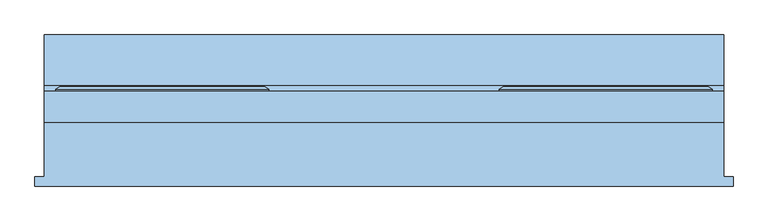
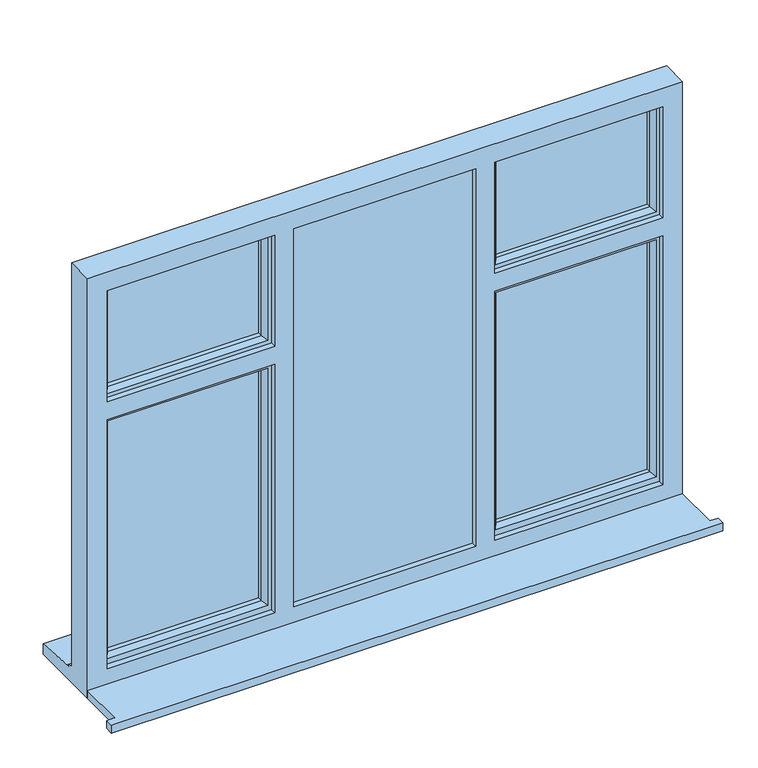
"""IFC4 building model written with IfcOpenShell, lengths in millimetres: window geometry, Window - Triple Casement with Top and Side Sashes : Window - Triple Casement with Top and Side Sashes."""

import ifcopenshell
import ifcopenshell.guid

model = None  # the IFC model being written
_history = None  # IfcOwnerHistory: only IFC2X3 demands one
_inside = {}  # id of a spatial element -> (the spatial element, [elements in it])
_under = {}  # id of a project, library or spatial element -> (it, [spatial elements below it])
_declared = {}  # id of a project -> (the project, [libraries it declares])
_typed = {}  # id of a type object -> (the type object, [elements of that type])
_made_of = {}  # id of a material, layer set ... -> (it, [elements and type objects made of it])


def new_model(schema):
    """Start an empty IFC model of exactly this schema.

    Asked for "IFC4X3", IfcOpenShell would pick the latest addendum, in which some entities
    have other attributes; the version numbers below select the first issue.
    IFC2X3 requires an IfcOwnerHistory on every rooted entity: one is made here for all.
    """
    global model, _history
    if schema == "IFC4X3":
        model = ifcopenshell.file(schema_version=(4, 3, 0, 0))
    else:
        model = ifcopenshell.file(schema=schema)
    _inside.clear()
    _under.clear()
    _declared.clear()
    _typed.clear()
    _made_of.clear()
    _history = None
    if model.schema == "IFC2X3":
        org = make("IfcOrganization", Name="unknown")
        user = make(
            "IfcPersonAndOrganization",
            ThePerson=make("IfcPerson", FamilyName="unknown"),
            TheOrganization=org,
        )
        app = make(
            "IfcApplication",
            ApplicationDeveloper=org,
            Version="unknown",
            ApplicationFullName="unknown",
            ApplicationIdentifier="unknown",
        )
        _history = make(
            "IfcOwnerHistory",
            OwningUser=user,
            OwningApplication=app,
            ChangeAction="ADDED",
            CreationDate=0,
        )
    return model


def make(cls, **values):
    """One entity of the class cls with the attributes given. An attribute that is None is left unset."""
    return model.create_entity(
        cls, **{name: value for name, value in values.items() if value is not None}
    )


def rooted(cls, **values):
    """An entity with a GlobalId (a new one), such as an element, a storey or a relation."""
    return make(cls, GlobalId=ifcopenshell.guid.new(), OwnerHistory=_history, **values)


def si_unit(unit_type, name, prefix=None):
    """IfcSIUnit, for example si_unit("LENGTHUNIT", "METRE", prefix="MILLI")."""
    return make("IfcSIUnit", UnitType=unit_type, Prefix=prefix, Name=name)


def assignment(units):
    """IfcUnitAssignment: the units of a project."""
    return None if units is None else make("IfcUnitAssignment", Units=units)


def point(xyz):
    """IfcCartesianPoint."""
    return None if xyz is None else make("IfcCartesianPoint", Coordinates=xyz)


def direction(xyz):
    """IfcDirection."""
    return None if xyz is None else make("IfcDirection", DirectionRatios=xyz)


def frame(location, z_axis=None, x_axis=None):
    """IfcAxis2Placement3D, a coordinate frame: its origin and axes. An axis left out is left unset."""
    return make(
        "IfcAxis2Placement3D",
        Location=point(location),
        Axis=direction(z_axis),
        RefDirection=direction(x_axis),
    )


def origin():
    """The frame at (0, 0, 0) with its axes left unset."""
    return frame((0.0, 0.0, 0.0))


def place(relative_to, where):
    """IfcLocalPlacement: puts the frame where relative to a parent placement (None: the world)."""
    return make(
        "IfcLocalPlacement", PlacementRelTo=relative_to, RelativePlacement=where
    )


def context(
    kind, dimensions, precision=None, world=None, true_north=None, identifier=None
):
    """IfcGeometricRepresentationContext, for example the 3D "Model" context."""
    return make(
        "IfcGeometricRepresentationContext",
        ContextIdentifier=identifier,
        ContextType=kind,
        CoordinateSpaceDimension=dimensions,
        Precision=precision,
        WorldCoordinateSystem=world,
        TrueNorth=true_north,
    )


def project(units=None, contexts=None):
    """IfcProject with its units and contexts."""
    return rooted(
        "IfcProject",
        Name="project",
        RepresentationContexts=contexts,
        UnitsInContext=assignment(units),
    )


def spatial(cls, under=None, at=None, **own):
    """A site, building, storey or space (cls), placed at a placement, below another one or the project."""
    s = rooted(cls, ObjectPlacement=at, **own)
    if under is not None:
        _under.setdefault(under.id(), (under, []))[1].append(s)
    return s


def polyline(points):
    """IfcPolyline through the points."""
    return make("IfcPolyline", Points=[point(p) for p in points])


def outline(outer, holes=None, kind="AREA"):
    """IfcArbitraryClosedProfileDef: a profile drawn as a closed curve; with holes, ...WithVoids."""
    if holes is None:
        return make("IfcArbitraryClosedProfileDef", ProfileType=kind, OuterCurve=outer)
    return make(
        "IfcArbitraryProfileDefWithVoids",
        ProfileType=kind,
        OuterCurve=outer,
        InnerCurves=holes,
    )


def extrude(swept, where, along, depth):
    """IfcExtrudedAreaSolid: the profile swept, set in the frame where, extruded along a direction by depth."""
    return make(
        "IfcExtrudedAreaSolid",
        SweptArea=swept,
        Position=where,
        ExtrudedDirection=direction(along),
        Depth=depth,
    )


def faces_of(points, faces, orient=None, outer=None):
    """IfcFace entities. A face is a list of loops; a loop is a list of indices into points, from 0.

    orient and outer hold one flag for each loop. By default every Orientation is true, the
    first loop of a face is its IfcFaceOuterBound and the others are IfcFaceBound.
    """
    made = []
    for i, loops in enumerate(faces):
        bounds = []
        for j, loop in enumerate(loops):
            is_outer = j == 0 if outer is None else outer[i][j]
            bounds.append(
                make(
                    "IfcFaceOuterBound" if is_outer else "IfcFaceBound",
                    Bound=make("IfcPolyLoop", Polygon=[points[k] for k in loop]),
                    Orientation=True if orient is None else orient[i][j],
                )
            )
        made.append(make("IfcFace", Bounds=bounds))
    return made


def faceted_brep(points, faces, orient=None, outer=None, voids=None):
    """IfcFacetedBrep: a solid bounded by flat faces; with voids (closed shells), ...WithVoids."""
    shared = [point(p) for p in points]
    hull = make("IfcClosedShell", CfsFaces=faces_of(shared, faces, orient, outer))
    if voids is None:
        return make("IfcFacetedBrep", Outer=hull)
    return make(
        "IfcFacetedBrepWithVoids",
        Outer=hull,
        Voids=[
            make(cls, CfsFaces=faces_of(shared, fs, o, b)) for cls, fs, o, b in voids
        ],
    )


def shape(context_of_items, identifier, shape_type, items):
    """IfcShapeRepresentation: the items that make up one representation, for example the "Body"."""
    return make(
        "IfcShapeRepresentation",
        ContextOfItems=context_of_items,
        RepresentationIdentifier=identifier,
        RepresentationType=shape_type,
        Items=items,
    )


def source(mapping_origin, context_of_items, identifier, shape_type, items):
    """IfcRepresentationMap: a shape defined once, which mapped items show again and again."""
    return make(
        "IfcRepresentationMap",
        MappingOrigin=mapping_origin,
        MappedRepresentation=shape(context_of_items, identifier, shape_type, items),
    )


def transform(
    local_origin,
    x_axis=None,
    y_axis=None,
    z_axis=None,
    scale=None,
    scale2=None,
    scale3=None,
    uniform=True,
):
    """IfcCartesianTransformationOperator3D, or its non-uniform kind. x_axis, y_axis, z_axis: its Axis1, 2, 3."""
    if uniform:
        return make(
            "IfcCartesianTransformationOperator3D",
            Axis1=direction(x_axis),
            Axis2=direction(y_axis),
            LocalOrigin=point(local_origin),
            Scale=scale,
            Axis3=direction(z_axis),
        )
    return make(
        "IfcCartesianTransformationOperator3DnonUniform",
        Axis1=direction(x_axis),
        Axis2=direction(y_axis),
        LocalOrigin=point(local_origin),
        Scale=scale,
        Axis3=direction(z_axis),
        Scale2=scale2,
        Scale3=scale3,
    )


def mapped(mapping_source, mapping_target):
    """IfcMappedItem: shows the shape of a source again, moved by a transform."""
    return make(
        "IfcMappedItem", MappingSource=mapping_source, MappingTarget=mapping_target
    )


def made_of(thing, what):
    """Note that an element or type object is made of a material, layer set ...; save() writes the relation."""
    if what is not None:
        _made_of.setdefault(what.id(), (what, []))[1].append(thing)
    return thing


def element(
    cls,
    number,
    at=None,
    inside=None,
    cuts=None,
    type_object=None,
    material=None,
    context=None,
    identifier="Body",
    shape_type=None,
    held_by="IfcProductDefinitionShape",
    body=None,
    shapes=None,
    **own,
):
    """One element of the class cls, such as IfcWall. Its Tag is "e" and its number.

    at: its placement. inside: the storey or other place that contains it. cuts: it is an
    opening in that element (IfcRelVoidsElement). A single representation is given by context,
    identifier, shape_type and body (its items); several are given by shapes. held_by: the class
    of the entity that holds the representations. save() writes the other relations.
    """
    e = rooted(cls, Tag="e%d" % number, ObjectPlacement=at, **own)
    if body is not None:
        shapes = [shape(context, identifier, shape_type, body)]
    if shapes is not None:
        e.Representation = make(held_by, Representations=shapes)
    if inside is not None:
        _inside.setdefault(inside.id(), (inside, []))[1].append(e)
    if cuts is not None:
        rooted(
            "IfcRelVoidsElement", RelatingBuildingElement=cuts, RelatedOpeningElement=e
        )
    if type_object is not None:
        _typed.setdefault(type_object.id(), (type_object, []))[1].append(e)
    return made_of(e, material)


def aggregate(whole, parts):
    """IfcRelAggregates: a whole, such as a stair, and the parts it consists of."""
    return rooted("IfcRelAggregates", RelatingObject=whole, RelatedObjects=parts)


def save(model, path):
    """Write the relations noted so far, then the file.

    IfcRelAggregates (storeys below a building ...), IfcRelContainedInSpatialStructure (elements
    in a storey), IfcRelDefinesByType, IfcRelAssociatesMaterial and IfcRelDeclares: one each for
    every whole, place, type object, material and project.
    """
    for whole, parts in _under.values():
        aggregate(whole, parts)
    for where, things in _inside.values():
        rooted(
            "IfcRelContainedInSpatialStructure",
            RelatedElements=things,
            RelatingStructure=where,
        )
    for kind, things in _typed.values():
        rooted("IfcRelDefinesByType", RelatedObjects=things, RelatingType=kind)
    for what, things in _made_of.values():
        rooted("IfcRelAssociatesMaterial", RelatedObjects=things, RelatingMaterial=what)
    for by, libraries in _declared.values():
        rooted("IfcRelDeclares", RelatingContext=by, RelatedDefinitions=libraries)
    model.write(path)


def window_e8f23823(model_context):
    return source(origin(), model_context, "Body", "SolidModel", [
        extrude(outline(polyline([(-1506.6666667, -182.7934322), (-1506.6666667, -157.7934322), (-1481.6666667, -157.7934322), (-1481.6666667, -13.2934322), (328.3333333, -13.2934322), (328.3333333, -157.7934322), (353.3333333, -157.7934322), (353.3333333, -182.7934322), (-1506.6666667, -182.7934322)])), frame((0.0, 0.0, 760.0), z_axis=(0.0, 0.0, 1.0), x_axis=(1.0, 0.0, 0.0)), (0.0, 0.0, 1.0), 25.0),
        extrude(outline(polyline([(823.0, -863.3333333), (823.0, -290.0), (2070.0, -290.0), (2070.0, -863.3333333), (823.0, -863.3333333)]), holes=[polyline([(2060.0, -853.3333333), (2060.0, -300.0), (833.0, -300.0), (833.0, -853.3333333), (2060.0, -853.3333333)])]), frame((0.0, 28.7065678, 0.0), z_axis=(0.0, 1.0, 0.0), x_axis=(0.0, 0.0, 1.0)), (0.0, 0.0, 1.0), 41.0),
        faceted_brep([(-1451.6666667, 69.7065678, 2080.0), (-1451.6666667, 75.4800705, 2080.0), (-1451.6666667, 75.4800705, 1665.0), (-1451.6666667, 69.7065678, 1665.0), (-1441.6666667, 4.7065678, 2070.0), (-1441.6666667, 69.7065678, 2070.0), (-1441.6666667, 69.7065678, 1675.0), (-1441.6666667, 4.7065678, 1675.0), (-1401.6666667, 19.1994677, 2030.0), (-1411.8147044, 4.7065678, 2040.1480377), (-1411.8147044, 4.7065678, 1704.8519623), (-1401.6666667, 19.1994677, 1715.0), (-1401.6666667, 33.7065678, 2030.0), (-1401.6666667, 33.7065678, 1715.0), (-1411.6666667, 57.7065678, 2040.0), (-1411.6666667, 33.7065678, 2040.0), (-1411.6666667, 33.7065678, 1705.0), (-1411.6666667, 57.7065678, 1705.0), (-1401.6666667, 75.4800705, 2030.0), (-1401.6666667, 57.7065678, 2030.0), (-1401.6666667, 57.7065678, 1715.0), (-1401.6666667, 75.4800705, 1715.0), (-1419.1124215, 81.2535732, 2047.4457548), (-1419.1124215, 81.2535732, 1697.5542452), (-1440.882057, 81.2535732, 2069.2153903), (-1440.882057, 81.2535732, 1675.7846097), (-883.3333333, 75.4800705, 1665.0), (-883.3333333, 69.7065678, 1665.0), (-893.3333333, 69.7065678, 1675.0), (-893.3333333, 4.7065678, 1675.0), (-923.1852956, 4.7065678, 1704.8519623), (-933.3333333, 19.1994677, 1715.0), (-933.3333333, 33.7065678, 1715.0), (-923.3333333, 33.7065678, 1705.0), (-923.3333333, 57.7065678, 1705.0), (-933.3333333, 57.7065678, 1715.0), (-933.3333333, 75.4800705, 1715.0), (-915.8875785, 81.2535732, 1697.5542452), (-894.117943, 81.2535732, 1675.7846097), (-883.3333333, 75.4800705, 2080.0), (-883.3333333, 69.7065678, 2080.0), (-893.3333333, 69.7065678, 2070.0), (-893.3333333, 4.7065678, 2070.0), (-923.1852956, 4.7065678, 2040.1480377), (-933.3333333, 19.1994677, 2030.0), (-933.3333333, 33.7065678, 2030.0), (-923.3333333, 33.7065678, 2040.0), (-923.3333333, 57.7065678, 2040.0), (-933.3333333, 57.7065678, 2030.0), (-933.3333333, 75.4800705, 2030.0), (-915.8875785, 81.2535732, 2047.4457548), (-894.117943, 81.2535732, 2069.2153903)], [[[0, 1, 2, 3]], [[4, 5, 6, 7]], [[8, 9, 10, 11]], [[12, 8, 11, 13]], [[14, 15, 16, 17]], [[18, 19, 20, 21]], [[22, 18, 21, 23]], [[1, 24, 25, 2]], [[3, 2, 26, 27]], [[7, 6, 28, 29]], [[11, 10, 30, 31]], [[13, 11, 31, 32]], [[17, 16, 33, 34]], [[21, 20, 35, 36]], [[23, 21, 36, 37]], [[2, 25, 38, 26]], [[27, 26, 39, 40]], [[29, 28, 41, 42]], [[31, 30, 43, 44]], [[32, 31, 44, 45]], [[34, 33, 46, 47]], [[36, 35, 48, 49]], [[37, 36, 49, 50]], [[26, 38, 51, 39]], [[40, 39, 1, 0]], [[3, 27, 40, 0], [5, 41, 28, 6]], [[42, 41, 5, 4]], [[7, 29, 42, 4], [9, 43, 30, 10]], [[44, 43, 9, 8]], [[45, 44, 8, 12]], [[15, 46, 33, 16], [13, 32, 45, 12]], [[47, 46, 15, 14]], [[17, 34, 47, 14], [19, 48, 35, 20]], [[49, 48, 19, 18]], [[50, 49, 18, 22]], [[24, 51, 38, 25], [23, 37, 50, 22]], [[39, 51, 24, 1]]]),
        faceted_brep([(-1451.6666667, 69.7065678, 1655.0), (-1451.6666667, 75.4800705, 1655.0), (-1451.6666667, 75.4800705, 813.0), (-1451.6666667, 69.7065678, 813.0), (-1441.6666667, 4.7065678, 1645.0), (-1441.6666667, 69.7065678, 1645.0), (-1441.6666667, 69.7065678, 823.0), (-1441.6666667, 4.7065678, 823.0), (-1401.6666667, 19.1994677, 1605.0), (-1411.8147044, 4.7065678, 1615.1480377), (-1411.8147044, 4.7065678, 852.8519623), (-1401.6666667, 19.1994677, 863.0), (-1401.6666667, 33.7065678, 1605.0), (-1401.6666667, 33.7065678, 863.0), (-1411.6666667, 57.7065678, 1615.0), (-1411.6666667, 33.7065678, 1615.0), (-1411.6666667, 33.7065678, 853.0), (-1411.6666667, 57.7065678, 853.0), (-1401.6666667, 75.4800705, 1605.0), (-1401.6666667, 57.7065678, 1605.0), (-1401.6666667, 57.7065678, 863.0), (-1401.6666667, 75.4800705, 863.0), (-1419.1124215, 81.2535732, 1622.4457548), (-1419.1124215, 81.2535732, 845.5542452), (-1440.882057, 81.2535732, 1644.2153903), (-1440.882057, 81.2535732, 823.7846097), (-883.3333333, 75.4800705, 813.0), (-883.3333333, 69.7065678, 813.0), (-893.3333333, 69.7065678, 823.0), (-893.3333333, 4.7065678, 823.0), (-923.1852956, 4.7065678, 852.8519623), (-933.3333333, 19.1994677, 863.0), (-933.3333333, 33.7065678, 863.0), (-923.3333333, 33.7065678, 853.0), (-923.3333333, 57.7065678, 853.0), (-933.3333333, 57.7065678, 863.0), (-933.3333333, 75.4800705, 863.0), (-915.8875785, 81.2535732, 845.5542452), (-894.117943, 81.2535732, 823.7846097), (-883.3333333, 75.4800705, 1655.0), (-883.3333333, 69.7065678, 1655.0), (-893.3333333, 69.7065678, 1645.0), (-893.3333333, 4.7065678, 1645.0), (-923.1852956, 4.7065678, 1615.1480377), (-933.3333333, 19.1994677, 1605.0), (-933.3333333, 33.7065678, 1605.0), (-923.3333333, 33.7065678, 1615.0), (-923.3333333, 57.7065678, 1615.0), (-933.3333333, 57.7065678, 1605.0), (-933.3333333, 75.4800705, 1605.0), (-915.8875785, 81.2535732, 1622.4457548), (-894.117943, 81.2535732, 1644.2153903)], [[[0, 1, 2, 3]], [[4, 5, 6, 7]], [[8, 9, 10, 11]], [[12, 8, 11, 13]], [[14, 15, 16, 17]], [[18, 19, 20, 21]], [[22, 18, 21, 23]], [[1, 24, 25, 2]], [[3, 2, 26, 27]], [[7, 6, 28, 29]], [[11, 10, 30, 31]], [[13, 11, 31, 32]], [[17, 16, 33, 34]], [[21, 20, 35, 36]], [[23, 21, 36, 37]], [[2, 25, 38, 26]], [[27, 26, 39, 40]], [[29, 28, 41, 42]], [[31, 30, 43, 44]], [[32, 31, 44, 45]], [[34, 33, 46, 47]], [[36, 35, 48, 49]], [[37, 36, 49, 50]], [[26, 38, 51, 39]], [[40, 39, 1, 0]], [[3, 27, 40, 0], [5, 41, 28, 6]], [[42, 41, 5, 4]], [[7, 29, 42, 4], [9, 43, 30, 10]], [[44, 43, 9, 8]], [[45, 44, 8, 12]], [[15, 46, 33, 16], [13, 32, 45, 12]], [[47, 46, 15, 14]], [[17, 34, 47, 14], [19, 48, 35, 20]], [[49, 48, 19, 18]], [[50, 49, 18, 22]], [[24, 51, 38, 25], [23, 37, 50, 22]], [[39, 51, 24, 1]]]),
        faceted_brep([(-270.0, 69.7065678, 2080.0), (-270.0, 75.4800705, 2080.0), (-270.0, 75.4800705, 1665.0), (-270.0, 69.7065678, 1665.0), (-260.0, 4.7065678, 2070.0), (-260.0, 69.7065678, 2070.0), (-260.0, 69.7065678, 1675.0), (-260.0, 4.7065678, 1675.0), (-220.0, 19.1994677, 2030.0), (-230.1480377, 4.7065678, 2040.1480377), (-230.1480377, 4.7065678, 1704.8519623), (-220.0, 19.1994677, 1715.0), (-220.0, 33.7065678, 2030.0), (-220.0, 33.7065678, 1715.0), (-230.0, 57.7065678, 2040.0), (-230.0, 33.7065678, 2040.0), (-230.0, 33.7065678, 1705.0), (-230.0, 57.7065678, 1705.0), (-220.0, 75.4800705, 2030.0), (-220.0, 57.7065678, 2030.0), (-220.0, 57.7065678, 1715.0), (-220.0, 75.4800705, 1715.0), (-237.4457548, 81.2535732, 2047.4457548), (-237.4457548, 81.2535732, 1697.5542452), (-259.2153903, 81.2535732, 2069.2153903), (-259.2153903, 81.2535732, 1675.7846097), (298.3333333, 75.4800705, 1665.0), (298.3333333, 69.7065678, 1665.0), (288.3333333, 69.7065678, 1675.0), (288.3333333, 4.7065678, 1675.0), (258.4813711, 4.7065678, 1704.8519623), (248.3333333, 19.1994677, 1715.0), (248.3333333, 33.7065678, 1715.0), (258.3333333, 33.7065678, 1705.0), (258.3333333, 57.7065678, 1705.0), (248.3333333, 57.7065678, 1715.0), (248.3333333, 75.4800705, 1715.0), (265.7790881, 81.2535732, 1697.5542452), (287.5487236, 81.2535732, 1675.7846097), (298.3333333, 75.4800705, 2080.0), (298.3333333, 69.7065678, 2080.0), (288.3333333, 69.7065678, 2070.0), (288.3333333, 4.7065678, 2070.0), (258.4813711, 4.7065678, 2040.1480377), (248.3333333, 19.1994677, 2030.0), (248.3333333, 33.7065678, 2030.0), (258.3333333, 33.7065678, 2040.0), (258.3333333, 57.7065678, 2040.0), (248.3333333, 57.7065678, 2030.0), (248.3333333, 75.4800705, 2030.0), (265.7790881, 81.2535732, 2047.4457548), (287.5487236, 81.2535732, 2069.2153903)], [[[0, 1, 2, 3]], [[4, 5, 6, 7]], [[8, 9, 10, 11]], [[12, 8, 11, 13]], [[14, 15, 16, 17]], [[18, 19, 20, 21]], [[22, 18, 21, 23]], [[1, 24, 25, 2]], [[3, 2, 26, 27]], [[7, 6, 28, 29]], [[11, 10, 30, 31]], [[13, 11, 31, 32]], [[17, 16, 33, 34]], [[21, 20, 35, 36]], [[23, 21, 36, 37]], [[2, 25, 38, 26]], [[27, 26, 39, 40]], [[29, 28, 41, 42]], [[31, 30, 43, 44]], [[32, 31, 44, 45]], [[34, 33, 46, 47]], [[36, 35, 48, 49]], [[37, 36, 49, 50]], [[26, 38, 51, 39]], [[40, 39, 1, 0]], [[3, 27, 40, 0], [5, 41, 28, 6]], [[42, 41, 5, 4]], [[7, 29, 42, 4], [9, 43, 30, 10]], [[44, 43, 9, 8]], [[45, 44, 8, 12]], [[15, 46, 33, 16], [13, 32, 45, 12]], [[47, 46, 15, 14]], [[17, 34, 47, 14], [19, 48, 35, 20]], [[49, 48, 19, 18]], [[50, 49, 18, 22]], [[24, 51, 38, 25], [23, 37, 50, 22]], [[39, 51, 24, 1]]]),
        extrude(outline(polyline([(258.3333333, 33.7065678), (-230.1480377, 33.7065678), (-230.1480377, 57.7065678), (258.3333333, 57.7065678), (258.3333333, 33.7065678)])), frame((0.0, 0.0, 852.8519623), z_axis=(0.0, 0.0, 1.0), x_axis=(1.0, 0.0, 0.0)), (0.0, 0.0, 1.0), 762.1480377),
        extrude(outline(polyline([(258.3333333, 33.7065678), (-230.0, 33.7065678), (-230.0, 57.7065678), (258.3333333, 57.7065678), (258.3333333, 33.7065678)])), frame((0.0, 0.0, 1705.0), z_axis=(0.0, 0.0, 1.0), x_axis=(1.0, 0.0, 0.0)), (0.0, 0.0, 1.0), 335.0),
        extrude(outline(polyline([(-923.3333333, 33.7065678), (-1411.6666667, 33.7065678), (-1411.6666667, 57.7065678), (-923.3333333, 57.7065678), (-923.3333333, 33.7065678)])), frame((0.0, 0.0, 1705.0), z_axis=(0.0, 0.0, 1.0), x_axis=(1.0, 0.0, 0.0)), (0.0, 0.0, 1.0), 335.0),
        extrude(outline(polyline([(-923.3333333, 33.7065678), (-1411.6666667, 33.7065678), (-1411.6666667, 57.7065678), (-923.3333333, 57.7065678), (-923.3333333, 33.7065678)])), frame((0.0, 0.0, 853.0), z_axis=(0.0, 0.0, 1.0), x_axis=(1.0, 0.0, 0.0)), (0.0, 0.0, 1.0), 762.0),
        faceted_brep([(-270.0, 69.7065678, 1655.0), (-270.0, 75.4800705, 1655.0), (-270.0, 75.4800705, 813.0), (-270.0, 69.7065678, 813.0), (-260.0, 4.7065678, 1645.0), (-260.0, 69.7065678, 1645.0), (-260.0, 69.7065678, 823.0), (-260.0, 4.7065678, 823.0), (-220.0, 19.1994677, 1605.0), (-230.1480377, 4.7065678, 1615.1480377), (-230.1480377, 4.7065678, 852.8519623), (-220.0, 19.1994677, 863.0), (-220.0, 33.7065678, 1605.0), (-220.0, 33.7065678, 863.0), (-230.0, 57.7065678, 1615.0), (-230.0, 33.7065678, 1615.0), (-230.0, 33.7065678, 853.0), (-230.0, 57.7065678, 853.0), (-220.0, 75.4800705, 1605.0), (-220.0, 57.7065678, 1605.0), (-220.0, 57.7065678, 863.0), (-220.0, 75.4800705, 863.0), (-237.4457548, 81.2535732, 1622.4457548), (-237.4457548, 81.2535732, 845.5542452), (-259.2153903, 81.2535732, 1644.2153903), (-259.2153903, 81.2535732, 823.7846097), (298.3333333, 75.4800705, 813.0), (298.3333333, 69.7065678, 813.0), (288.3333333, 69.7065678, 823.0), (288.3333333, 4.7065678, 823.0), (258.4813711, 4.7065678, 852.8519623), (248.3333333, 19.1994677, 863.0), (248.3333333, 33.7065678, 863.0), (258.3333333, 33.7065678, 853.0), (258.3333333, 57.7065678, 853.0), (248.3333333, 57.7065678, 863.0), (248.3333333, 75.4800705, 863.0), (265.7790881, 81.2535732, 845.5542452), (287.5487236, 81.2535732, 823.7846097), (298.3333333, 75.4800705, 1655.0), (298.3333333, 69.7065678, 1655.0), (288.3333333, 69.7065678, 1645.0), (288.3333333, 4.7065678, 1645.0), (258.4813711, 4.7065678, 1615.1480377), (248.3333333, 19.1994677, 1605.0), (248.3333333, 33.7065678, 1605.0), (258.3333333, 33.7065678, 1615.0), (258.3333333, 57.7065678, 1615.0), (248.3333333, 57.7065678, 1605.0), (248.3333333, 75.4800705, 1605.0), (265.7790881, 81.2535732, 1622.4457548), (287.5487236, 81.2535732, 1644.2153903)], [[[0, 1, 2, 3]], [[4, 5, 6, 7]], [[8, 9, 10, 11]], [[12, 8, 11, 13]], [[14, 15, 16, 17]], [[18, 19, 20, 21]], [[22, 18, 21, 23]], [[1, 24, 25, 2]], [[3, 2, 26, 27]], [[7, 6, 28, 29]], [[11, 10, 30, 31]], [[13, 11, 31, 32]], [[17, 16, 33, 34]], [[21, 20, 35, 36]], [[23, 21, 36, 37]], [[2, 25, 38, 26]], [[27, 26, 39, 40]], [[29, 28, 41, 42]], [[31, 30, 43, 44]], [[32, 31, 44, 45]], [[34, 33, 46, 47]], [[36, 35, 48, 49]], [[37, 36, 49, 50]], [[26, 38, 51, 39]], [[40, 39, 1, 0]], [[3, 27, 40, 0], [5, 41, 28, 6]], [[42, 41, 5, 4]], [[7, 29, 42, 4], [9, 43, 30, 10]], [[44, 43, 9, 8]], [[45, 44, 8, 12]], [[15, 46, 33, 16], [13, 32, 45, 12]], [[47, 46, 15, 14]], [[17, 34, 47, 14], [19, 48, 35, 20]], [[49, 48, 19, 18]], [[50, 49, 18, 22]], [[24, 51, 38, 25], [23, 37, 50, 22]], [[39, 51, 24, 1]]]),
        faceted_brep([(328.3333333, -13.2934322, 2110.0), (-1481.6666667, -13.2934322, 2110.0), (-1481.6666667, -13.2934322, 760.0), (328.3333333, -13.2934322, 760.0), (268.3333333, -13.2934322, 835.0), (-242.0, -13.2934322, 835.0), (-242.0, -13.2934322, 1635.0), (268.3333333, -13.2934322, 1635.0), (-853.3333333, -13.2934322, 2050.0), (-300.0, -13.2934322, 2050.0), (-300.0, -13.2934322, 835.0), (-853.3333333, -13.2934322, 835.0), (-242.0, -13.2934322, 2050.0), (268.3333333, -13.2934322, 2050.0), (268.3333333, -13.2934322, 1693.0), (-242.0, -13.2934322, 1693.0), (-1421.6666667, -13.2934322, 835.0), (-1421.6666667, -13.2934322, 1635.0), (-911.3333333, -13.2934322, 1635.0), (-911.3333333, -13.2934322, 835.0), (-1421.6666667, -13.2934322, 2050.0), (-911.3333333, -13.2934322, 2050.0), (-911.3333333, -13.2934322, 1693.0), (-1421.6666667, -13.2934322, 1693.0), (-1481.6666667, 69.7065678, 2110.0), (-1481.6666667, 69.7065678, 811.0), (-1481.6666667, 84.7065678, 809.68767), (-1481.6666667, 84.7065678, 804.7449676), (-1481.6666667, 219.7065678, 793.8088847), (-1481.6666667, 219.7065678, 760.0), (328.3333333, 69.7065678, 2110.0), (328.3333333, 69.7065678, 811.0), (-260.0, 69.7065678, 823.0), (288.3333333, 69.7065678, 823.0), (288.3333333, 69.7065678, 1645.0), (-260.0, 69.7065678, 1645.0), (288.3333333, 69.7065678, 2070.0), (-260.0, 69.7065678, 2070.0), (-260.0, 69.7065678, 1675.0), (288.3333333, 69.7065678, 1675.0), (-893.3333333, 69.7065678, 823.0), (-893.3333333, 69.7065678, 1645.0), (-1441.6666667, 69.7065678, 1645.0), (-1441.6666667, 69.7065678, 823.0), (-893.3333333, 69.7065678, 2070.0), (-1441.6666667, 69.7065678, 2070.0), (-1441.6666667, 69.7065678, 1675.0), (-893.3333333, 69.7065678, 1675.0), (-853.3333333, 69.7065678, 2070.0), (-853.3333333, 69.7065678, 823.0), (-300.0, 69.7065678, 823.0), (-300.0, 69.7065678, 2070.0), (-1441.6666667, 4.7065678, 2070.0), (-1441.6666667, 4.7065678, 1675.0), (-1441.6666667, 4.7065678, 1645.0), (-1441.6666667, 4.7065678, 823.0), (-893.3333333, 4.7065678, 2070.0), (-893.3333333, 4.7065678, 1675.0), (-911.3333333, 4.7065678, 2050.0), (-1421.6666667, 4.7065678, 2050.0), (-1421.6666667, 4.7065678, 1693.0), (-911.3333333, 4.7065678, 1693.0), (-260.0, 4.7065678, 2070.0), (288.3333333, 4.7065678, 2070.0), (288.3333333, 4.7065678, 1675.0), (-260.0, 4.7065678, 1675.0), (268.3333333, 4.7065678, 2050.0), (-242.0, 4.7065678, 2050.0), (-242.0, 4.7065678, 1693.0), (268.3333333, 4.7065678, 1693.0), (-863.3333333, 4.7065678, 2070.0), (-290.0, 4.7065678, 2070.0), (-290.0, 4.7065678, 823.0), (-863.3333333, 4.7065678, 823.0), (-300.0, 4.7065678, 2050.0), (-853.3333333, 4.7065678, 2050.0), (-853.3333333, 4.7065678, 835.0), (-300.0, 4.7065678, 835.0), (-893.3333333, 4.7065678, 823.0), (-893.3333333, 4.7065678, 1645.0), (-1421.6666667, 4.7065678, 835.0), (-911.3333333, 4.7065678, 835.0), (-911.3333333, 4.7065678, 1635.0), (-1421.6666667, 4.7065678, 1635.0), (288.3333333, 4.7065678, 823.0), (-260.0, 4.7065678, 823.0), (-260.0, 4.7065678, 1645.0), (288.3333333, 4.7065678, 1645.0), (-242.0, 4.7065678, 835.0), (268.3333333, 4.7065678, 835.0), (268.3333333, 4.7065678, 1635.0), (-242.0, 4.7065678, 1635.0), (-853.3333333, 28.7065678, 2070.0), (-300.0, 28.7065678, 2070.0), (-290.0, 28.7065678, 2070.0), (-863.3333333, 28.7065678, 2070.0), (328.3333333, 219.7065678, 760.0), (328.3333333, 219.7065678, 793.8088847), (328.3333333, 84.7065678, 804.7449676), (328.3333333, 84.7065678, 809.68767), (-853.3333333, 28.7065678, 823.0), (-863.3333333, 28.7065678, 823.0), (-290.0, 28.7065678, 823.0), (-300.0, 28.7065678, 823.0)], [[[0, 1, 2, 3], [4, 5, 6, 7], [8, 9, 10, 11], [12, 13, 14, 15], [16, 17, 18, 19], [20, 21, 22, 23]], [[1, 24, 25, 26, 27, 28, 29, 2]], [[24, 30, 31, 25], [32, 33, 34, 35], [36, 37, 38, 39], [40, 41, 42, 43], [44, 45, 46, 47], [48, 49, 50, 51]], [[45, 52, 53, 46]], [[54, 55, 43, 42]], [[52, 56, 57, 53], [58, 59, 60, 61]], [[62, 63, 64, 65], [66, 67, 68, 69]], [[70, 71, 72, 73], [74, 75, 76, 77]], [[78, 55, 54, 79], [80, 81, 82, 83]], [[84, 85, 86, 87], [88, 89, 90, 91]], [[59, 20, 23, 60]], [[16, 80, 83, 17]], [[1, 0, 30, 24]], [[52, 45, 44, 56]], [[36, 63, 62, 37]], [[92, 48, 51, 93, 94, 71, 70, 95]], [[20, 59, 58, 21]], [[66, 13, 12, 67]], [[8, 75, 74, 9]], [[30, 0, 3, 96, 97, 98, 99, 31]], [[63, 36, 39, 64]], [[33, 84, 87, 34]], [[13, 66, 69, 14]], [[89, 4, 7, 90]], [[75, 8, 11, 76]], [[21, 58, 61, 22]], [[81, 19, 18, 82]], [[57, 56, 44, 47]], [[40, 78, 79, 41]], [[49, 48, 92, 100]], [[100, 92, 95, 101]], [[101, 95, 70, 73]], [[94, 102, 72, 71]], [[102, 94, 93, 103]], [[103, 93, 51, 50]], [[37, 62, 65, 38]], [[85, 32, 35, 86]], [[67, 12, 15, 68]], [[5, 88, 91, 6]], [[9, 74, 77, 10]], [[96, 3, 2, 29]], [[97, 96, 29, 28]], [[98, 97, 28, 27]], [[99, 98, 27, 26]], [[31, 99, 26, 25]], [[33, 32, 85, 84]], [[40, 43, 55, 78]], [[50, 49, 100, 101, 73, 72, 102, 103]], [[5, 4, 89, 88]], [[77, 76, 11, 10]], [[81, 80, 16, 19]], [[35, 34, 87, 86]], [[39, 38, 65, 64]], [[15, 14, 69, 68]], [[7, 6, 91, 90]], [[47, 46, 53, 57]], [[42, 41, 79, 54]], [[83, 82, 18, 17]], [[61, 60, 23, 22]]]),
        extrude(outline(polyline([(-863.3333333, 28.7065678), (-290.0, 28.7065678), (-290.0, 4.7065678), (-863.3333333, 4.7065678), (-863.3333333, 28.7065678)])), frame((0.0, 0.0, 823.0), z_axis=(0.0, 0.0, 1.0), x_axis=(1.0, 0.0, 0.0)), (0.0, 0.0, 1.0), 1247.0),
    ])


if __name__ == "__main__":
    model = new_model("IFC4")
    model_context = context("Model", 3, world=origin())
    ifc_project = project(units=[si_unit("LENGTHUNIT", "METRE", prefix="MILLI")], contexts=[model_context])
    site = spatial("IfcSite", under=ifc_project)
    building = spatial("IfcBuilding", under=site)
    placement = place(None, origin())
    window_shape = window_e8f23823(model_context)
    element("IfcWindow", 1, ObjectType="Window - Triple Casement with Top and Side Sashes : Window - Triple Casement with Top and Side Sashes", at=placement, inside=building, context=model_context, shape_type="MappedRepresentation", body=[
        mapped(window_shape, transform((0.0, 0.0, 0.0), x_axis=(1.0, 0.0, 0.0), y_axis=(0.0, 1.0, 0.0), z_axis=(0.0, 0.0, 1.0))),
    ])
    save(model, "model.ifc")

# Revit data of these elements
# Type "Window - Triple Casement with Top and Side Sashes : Window - Triple Casement with Top and Side Sashes"
#   Description = "Triple Casement Window with Opening Sash Vents"
#   Type Mark = "51"
#   Operation = "Userdefined"
#   Manufacturer = "Revit"
#   Keynote = "L10"
#   Wrap Layers (Ext) from Ext = 100 mm
#   Wrap Layers (Int) from Ext = 177.5 mm
#   Window Board Projection = 25 mm
#   Window Board Extension = 25 mm
#   Visual Light Transmittance = 0.9
#   Vent Height = 450 mm
#   Solar Heat Gain Coefficient = 0.78
#   Rough Width = 1810 mm
#   Rough Height = 1350 mm
#   Height = 1350 mm
#   Width = 1810 mm
#   Heat Transfer Coefficient (U) = 3.6886 W/(m²·K)
#   Glazing Thickness = 24 mm
#   FrameOffset - External = 105 mm
#   Frame Depth = 65 mm
#   Default Head Height = 2110 mm
#   Cill Depth = 150 mm
#   Cavity Closer Width = 50 mm
#   Cavity Closer Offset from Ext = 102.5 mm
#   Cavity Closer Depth = 85 mm
#   Vis - Cavity Closers = yes
#   Define Thermal Properties by = 1
#   Material Trim = Window Frame
#   Material Glass = Glass
#   Material Frame = Window Frame
#   Construction Type Id = ""
#   Wall Closure = (empty or 0)
#   Analytic Construction = (empty or 0)
# Element 1 (IfcWindow, "Window - Triple Casement with Top and Side Sashes : Window - Triple Casement with Top and Side Sashes")
#   Materials on its faces: "Window Frame", "Glass"
# Materials
#   "Window Frame": class "Miscellaneous", colour RGB 249 249 249, transparency 0, Keynote = "L10"
#   "Glass": class "Glass", colour RGB 0 128 192, transparency 0.9, Description = "Soda Lime Glass", Cost = 0
